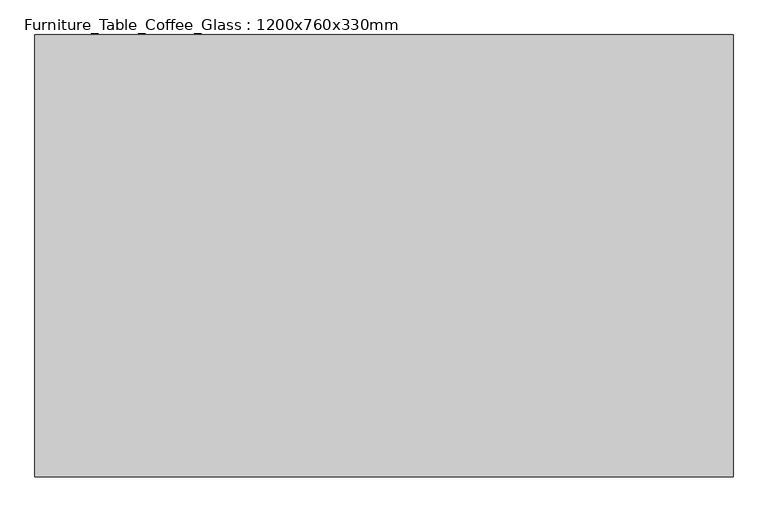
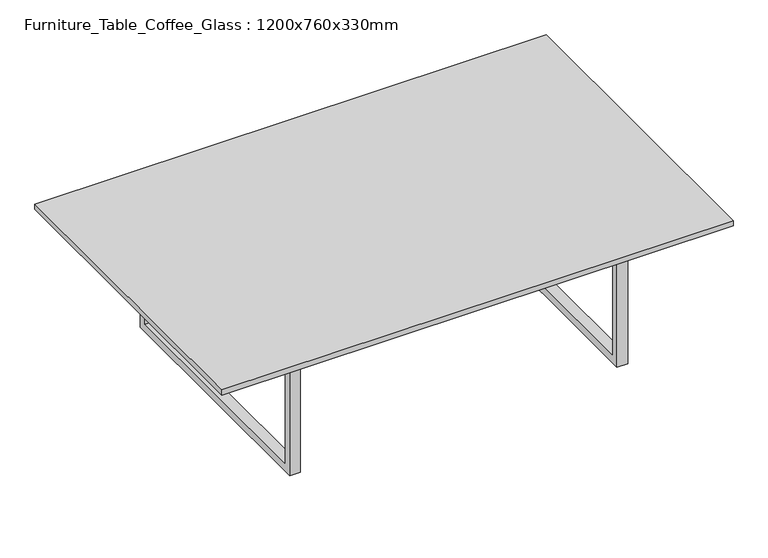
"""IFC4 building model written with IfcOpenShell, lengths in millimetres: furniture geometry, Furniture_Table_Coffee_Glass : 1200x760x330mm."""

import ifcopenshell
import ifcopenshell.guid

model = None  # the IFC model being written
_history = None  # IfcOwnerHistory: only IFC2X3 demands one
_inside = {}  # id of a spatial element -> (the spatial element, [elements in it])
_under = {}  # id of a project, library or spatial element -> (it, [spatial elements below it])
_declared = {}  # id of a project -> (the project, [libraries it declares])
_typed = {}  # id of a type object -> (the type object, [elements of that type])
_made_of = {}  # id of a material, layer set ... -> (it, [elements and type objects made of it])


def new_model(schema):
    """Start an empty IFC model of exactly this schema.

    Asked for "IFC4X3", IfcOpenShell would pick the latest addendum, in which some entities
    have other attributes; the version numbers below select the first issue.
    IFC2X3 requires an IfcOwnerHistory on every rooted entity: one is made here for all.
    """
    global model, _history
    if schema == "IFC4X3":
        model = ifcopenshell.file(schema_version=(4, 3, 0, 0))
    else:
        model = ifcopenshell.file(schema=schema)
    _inside.clear()
    _under.clear()
    _declared.clear()
    _typed.clear()
    _made_of.clear()
    _history = None
    if model.schema == "IFC2X3":
        org = make("IfcOrganization", Name="unknown")
        user = make(
            "IfcPersonAndOrganization",
            ThePerson=make("IfcPerson", FamilyName="unknown"),
            TheOrganization=org,
        )
        app = make(
            "IfcApplication",
            ApplicationDeveloper=org,
            Version="unknown",
            ApplicationFullName="unknown",
            ApplicationIdentifier="unknown",
        )
        _history = make(
            "IfcOwnerHistory",
            OwningUser=user,
            OwningApplication=app,
            ChangeAction="ADDED",
            CreationDate=0,
        )
    return model


def make(cls, **values):
    """One entity of the class cls with the attributes given. An attribute that is None is left unset."""
    return model.create_entity(
        cls, **{name: value for name, value in values.items() if value is not None}
    )


def rooted(cls, **values):
    """An entity with a GlobalId (a new one), such as an element, a storey or a relation."""
    return make(cls, GlobalId=ifcopenshell.guid.new(), OwnerHistory=_history, **values)


def si_unit(unit_type, name, prefix=None):
    """IfcSIUnit, for example si_unit("LENGTHUNIT", "METRE", prefix="MILLI")."""
    return make("IfcSIUnit", UnitType=unit_type, Prefix=prefix, Name=name)


def assignment(units):
    """IfcUnitAssignment: the units of a project."""
    return None if units is None else make("IfcUnitAssignment", Units=units)


def point(xyz):
    """IfcCartesianPoint."""
    return None if xyz is None else make("IfcCartesianPoint", Coordinates=xyz)


def direction(xyz):
    """IfcDirection."""
    return None if xyz is None else make("IfcDirection", DirectionRatios=xyz)


def frame(location, z_axis=None, x_axis=None):
    """IfcAxis2Placement3D, a coordinate frame: its origin and axes. An axis left out is left unset."""
    return make(
        "IfcAxis2Placement3D",
        Location=point(location),
        Axis=direction(z_axis),
        RefDirection=direction(x_axis),
    )


def origin():
    """The frame at (0, 0, 0) with its axes left unset."""
    return frame((0.0, 0.0, 0.0))


def place(relative_to, where):
    """IfcLocalPlacement: puts the frame where relative to a parent placement (None: the world)."""
    return make(
        "IfcLocalPlacement", PlacementRelTo=relative_to, RelativePlacement=where
    )


def context(
    kind, dimensions, precision=None, world=None, true_north=None, identifier=None
):
    """IfcGeometricRepresentationContext, for example the 3D "Model" context."""
    return make(
        "IfcGeometricRepresentationContext",
        ContextIdentifier=identifier,
        ContextType=kind,
        CoordinateSpaceDimension=dimensions,
        Precision=precision,
        WorldCoordinateSystem=world,
        TrueNorth=true_north,
    )


def project(units=None, contexts=None):
    """IfcProject with its units and contexts."""
    return rooted(
        "IfcProject",
        Name="project",
        RepresentationContexts=contexts,
        UnitsInContext=assignment(units),
    )


def spatial(cls, under=None, at=None, **own):
    """A site, building, storey or space (cls), placed at a placement, below another one or the project."""
    s = rooted(cls, ObjectPlacement=at, **own)
    if under is not None:
        _under.setdefault(under.id(), (under, []))[1].append(s)
    return s


def polyline(points):
    """IfcPolyline through the points."""
    return make("IfcPolyline", Points=[point(p) for p in points])


def outline(outer, holes=None, kind="AREA"):
    """IfcArbitraryClosedProfileDef: a profile drawn as a closed curve; with holes, ...WithVoids."""
    if holes is None:
        return make("IfcArbitraryClosedProfileDef", ProfileType=kind, OuterCurve=outer)
    return make(
        "IfcArbitraryProfileDefWithVoids",
        ProfileType=kind,
        OuterCurve=outer,
        InnerCurves=holes,
    )


def extrude(swept, where, along, depth):
    """IfcExtrudedAreaSolid: the profile swept, set in the frame where, extruded along a direction by depth."""
    return make(
        "IfcExtrudedAreaSolid",
        SweptArea=swept,
        Position=where,
        ExtrudedDirection=direction(along),
        Depth=depth,
    )


def shape(context_of_items, identifier, shape_type, items):
    """IfcShapeRepresentation: the items that make up one representation, for example the "Body"."""
    return make(
        "IfcShapeRepresentation",
        ContextOfItems=context_of_items,
        RepresentationIdentifier=identifier,
        RepresentationType=shape_type,
        Items=items,
    )


def source(mapping_origin, context_of_items, identifier, shape_type, items):
    """IfcRepresentationMap: a shape defined once, which mapped items show again and again."""
    return make(
        "IfcRepresentationMap",
        MappingOrigin=mapping_origin,
        MappedRepresentation=shape(context_of_items, identifier, shape_type, items),
    )


def transform(
    local_origin,
    x_axis=None,
    y_axis=None,
    z_axis=None,
    scale=None,
    scale2=None,
    scale3=None,
    uniform=True,
):
    """IfcCartesianTransformationOperator3D, or its non-uniform kind. x_axis, y_axis, z_axis: its Axis1, 2, 3."""
    if uniform:
        return make(
            "IfcCartesianTransformationOperator3D",
            Axis1=direction(x_axis),
            Axis2=direction(y_axis),
            LocalOrigin=point(local_origin),
            Scale=scale,
            Axis3=direction(z_axis),
        )
    return make(
        "IfcCartesianTransformationOperator3DnonUniform",
        Axis1=direction(x_axis),
        Axis2=direction(y_axis),
        LocalOrigin=point(local_origin),
        Scale=scale,
        Axis3=direction(z_axis),
        Scale2=scale2,
        Scale3=scale3,
    )


def mapped(mapping_source, mapping_target):
    """IfcMappedItem: shows the shape of a source again, moved by a transform."""
    return make(
        "IfcMappedItem", MappingSource=mapping_source, MappingTarget=mapping_target
    )


def made_of(thing, what):
    """Note that an element or type object is made of a material, layer set ...; save() writes the relation."""
    if what is not None:
        _made_of.setdefault(what.id(), (what, []))[1].append(thing)
    return thing


def element(
    cls,
    number,
    at=None,
    inside=None,
    cuts=None,
    type_object=None,
    material=None,
    context=None,
    identifier="Body",
    shape_type=None,
    held_by="IfcProductDefinitionShape",
    body=None,
    shapes=None,
    **own,
):
    """One element of the class cls, such as IfcWall. Its Tag is "e" and its number.

    at: its placement. inside: the storey or other place that contains it. cuts: it is an
    opening in that element (IfcRelVoidsElement). A single representation is given by context,
    identifier, shape_type and body (its items); several are given by shapes. held_by: the class
    of the entity that holds the representations. save() writes the other relations.
    """
    e = rooted(cls, Tag="e%d" % number, ObjectPlacement=at, **own)
    if body is not None:
        shapes = [shape(context, identifier, shape_type, body)]
    if shapes is not None:
        e.Representation = make(held_by, Representations=shapes)
    if inside is not None:
        _inside.setdefault(inside.id(), (inside, []))[1].append(e)
    if cuts is not None:
        rooted(
            "IfcRelVoidsElement", RelatingBuildingElement=cuts, RelatedOpeningElement=e
        )
    if type_object is not None:
        _typed.setdefault(type_object.id(), (type_object, []))[1].append(e)
    return made_of(e, material)


def aggregate(whole, parts):
    """IfcRelAggregates: a whole, such as a stair, and the parts it consists of."""
    return rooted("IfcRelAggregates", RelatingObject=whole, RelatedObjects=parts)


def save(model, path):
    """Write the relations noted so far, then the file.

    IfcRelAggregates (storeys below a building ...), IfcRelContainedInSpatialStructure (elements
    in a storey), IfcRelDefinesByType, IfcRelAssociatesMaterial and IfcRelDeclares: one each for
    every whole, place, type object, material and project.
    """
    for whole, parts in _under.values():
        aggregate(whole, parts)
    for where, things in _inside.values():
        rooted(
            "IfcRelContainedInSpatialStructure",
            RelatedElements=things,
            RelatingStructure=where,
        )
    for kind, things in _typed.values():
        rooted("IfcRelDefinesByType", RelatedObjects=things, RelatingType=kind)
    for what, things in _made_of.values():
        rooted("IfcRelAssociatesMaterial", RelatedObjects=things, RelatingMaterial=what)
    for by, libraries in _declared.values():
        rooted("IfcRelDeclares", RelatingContext=by, RelatedDefinitions=libraries)
    model.write(path)


def furniture_table_coffee_glass_1200x760x330mm_c221341c(model_context):
    return source(origin(), model_context, "Body", "SweptSolid", [
        extrude(outline(polyline([(975.1336303, 378.1358318), (975.1336303, 359.0858318), (232.3336303, 359.0858318), (232.3336303, 378.1358318), (975.1336303, 378.1358318)])), frame((0.0, 0.0, 298.25), z_axis=(0.0, 0.0, 1.0), x_axis=(1.0, 0.0, 0.0)), (0.0, 0.0, 1.0), 19.05),
        extrude(outline(polyline([(64.8108318, 317.3), (672.4108318, 317.3), (672.4108318, 0.0), (64.8108318, 0.0), (64.8108318, 317.3)]), holes=[polyline([(83.8608318, 298.25), (83.8608318, 19.05), (653.3608318, 19.05), (653.3608318, 298.25), (83.8608318, 298.25)])]), frame((975.1336303, 0.0, 0.0), z_axis=(1.0, 0.0, 0.0), x_axis=(0.0, 1.0, 0.0)), (0.0, 0.0, 1.0), 25.4),
        extrude(outline(polyline([(64.8108318, 317.3), (672.4108318, 317.3), (672.4108318, 0.0), (64.8108318, 0.0), (64.8108318, 317.3)]), holes=[polyline([(83.8608318, 298.25), (83.8608318, 19.05), (653.3608318, 19.05), (653.3608318, 298.25), (83.8608318, 298.25)])]), frame((206.9336303, 0.0, 0.0), z_axis=(1.0, 0.0, 0.0), x_axis=(0.0, 1.0, 0.0)), (0.0, 0.0, 1.0), 25.4),
        extrude(outline(polyline([(1203.7336303, 748.6108318), (1203.7336303, -11.3891682), (3.7336303, -11.3891682), (3.7336303, 748.6108318), (1203.7336303, 748.6108318)])), frame((0.0, 0.0, 317.3), z_axis=(0.0, 0.0, 1.0), x_axis=(1.0, 0.0, 0.0)), (0.0, 0.0, 1.0), 12.7),
    ])


if __name__ == "__main__":
    model = new_model("IFC4")
    model_context = context("Model", 3, world=origin())
    ifc_project = project(units=[si_unit("LENGTHUNIT", "METRE", prefix="MILLI")], contexts=[model_context])
    site = spatial("IfcSite", under=ifc_project)
    building = spatial("IfcBuilding", under=site)
    placement = place(None, origin())
    furniture_table_coffee_glass_1200x760x330mm_shape = furniture_table_coffee_glass_1200x760x330mm_c221341c(model_context)
    element("IfcFurniture", 1, ObjectType="Furniture_Table_Coffee_Glass : 1200x760x330mm", at=placement, inside=building, context=model_context, shape_type="MappedRepresentation", body=[
        mapped(furniture_table_coffee_glass_1200x760x330mm_shape, transform((0.0, 0.0, 0.0), x_axis=(1.0, 0.0, 0.0), y_axis=(0.0, 1.0, 0.0), z_axis=(0.0, 0.0, 1.0))),
    ])
    save(model, "model.ifc")

# Revit data of these elements
# Type "Furniture_Table_Coffee_Glass : 1200x760x330mm"
#   Keynote = "N"
#   Height = 330 mm
#   Length = 1200 mm
#   Width = 760 mm
#   Material Base = Metal - Chrome
#   Material Top = Glass - Clear, Grey
#   Default Elevation = 0
#   Assembly Code = ""
# Element 1 (IfcFurniture, "Furniture_Table_Coffee_Glass : 1200x760x330mm")
#   Materials on its faces: "Metal - Chrome", "Glass - Clear, Grey"
# Materials
#   "Metal - Chrome": class "Metal", colour RGB 206 206 206, transparency 0
#   "Glass - Clear, Grey": class "Glass", colour RGB 252 255 255, transparency 0.64
